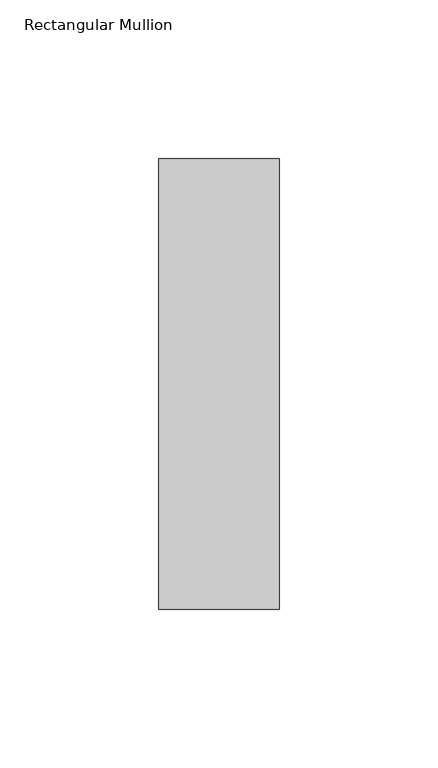
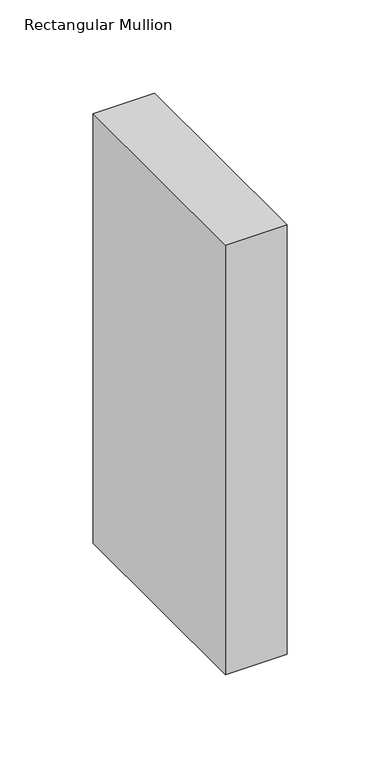
"""IFC4 building model written with IfcOpenShell, lengths in millimetres: member geometry, Rectangular Mullion : NLRS_21_CWM_hsb-regel 38x142_gen_rsf."""

from ifc_helpers import new_model, si_unit, frame, origin, place, context, project, spatial, polyline, outline, extrude, source, transform, mapped, element, save


def rectangular_mullion_8622cd22(model_context):
    return source(origin(), model_context, "Body", "SweptSolid", [
        extrude(outline(polyline([(0.0, -71.0), (-38.0, -71.0), (-38.0, 71.0), (0.0, 71.0), (0.0, -71.0)])), frame((0.0, 0.0, -280.9999997), z_axis=(0.0, 0.0, 1.0), x_axis=(1.0, 0.0, 0.0)), (0.0, 0.0, 1.0), 280.9999997),
    ])


if __name__ == "__main__":
    model = new_model("IFC4")
    model_context = context("Model", 3, world=origin())
    ifc_project = project(units=[si_unit("LENGTHUNIT", "METRE", prefix="MILLI")], contexts=[model_context])
    site = spatial("IfcSite", under=ifc_project)
    building = spatial("IfcBuilding", under=site)
    placement = place(None, origin())
    rectangular_mullion_shape = rectangular_mullion_8622cd22(model_context)
    element("IfcMember", 1, ObjectType="Rectangular Mullion : NLRS_21_CWM_hsb-regel 38x142_gen_rsf", at=placement, inside=building, context=model_context, shape_type="MappedRepresentation", body=[
        mapped(rectangular_mullion_shape, transform((0.0, 0.0, 0.0), x_axis=(1.0, 0.0, 0.0), y_axis=(0.0, 1.0, 0.0), z_axis=(0.0, 0.0, 1.0))),
    ])
    save(model, "model.ifc")

# Revit data of these elements
# Type "Rectangular Mullion : NLRS_21_CWM_hsb-regel 38x142_gen_rsf"
#   Export Type to IFC As = "IfcWall"
#   Type IfcGUID = "07M7mRoiH1CR8m_RSKIwpF"
#   Assembly Code = "21.10"
#   built-in parameter 1007322 = 0.465879 (stored number, unit not read)
#   built-in parameter 1007321 = 0.062336 (stored number, unit not read)
#   built-in parameter 1007320 = 0.062336 (stored number, unit not read)
# Element 1 (IfcMember, "Rectangular Mullion : NLRS_21_CWM_hsb-regel 38x142_gen_rsf")
#   Materials on its faces: "NLRS_i2_hout naaldhout vuren_gen_rsf"
# Materials
#   "NLRS_i2_hout naaldhout vuren_gen_rsf": class "I - Hout", colour RGB 234 199 147, transparency 0, Keynote = "i2", Manufacturer = "Revit Standards Foundation", URL = "www.revitstandards.org", Description = "hout vuren", Cost = 0
